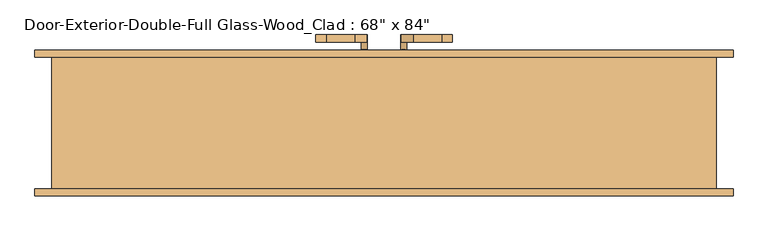
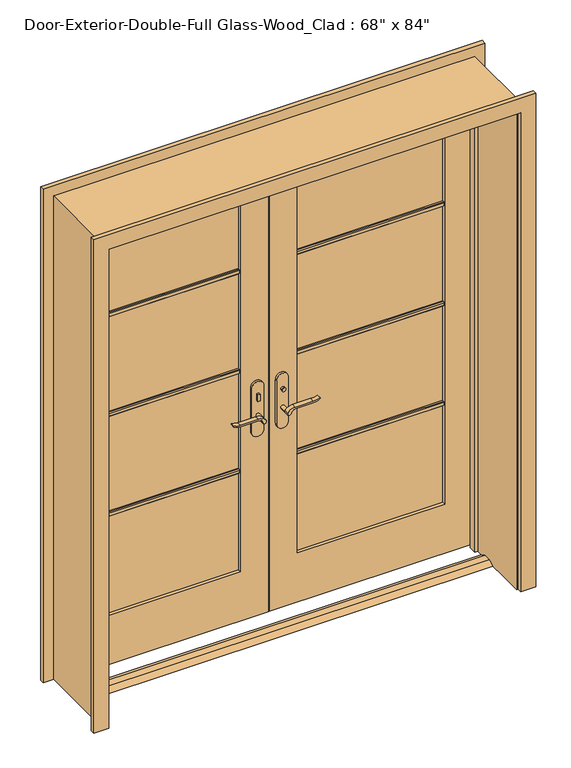
"""IFC4 building model written with IfcOpenShell, lengths in millimetres: door geometry."""

from ifc_helpers import new_model, si_unit, point, frame, frame_2d, origin, place, context, project, spatial, polyline, circle_curve, trimmed, segment, composite_curve, outline, extrude, faceted_brep, source, transform, mapped, element, save


def door_f2de18c9(model_context):
    return source(origin(), model_context, "Body", "SolidModel", [
        extrude(outline(polyline([(19.05, 12.7), (53.975, 12.7), (79.375, 0.0), (-6.35, 0.0), (19.05, 12.7)])), frame((-863.6, 0.0, 0.0), z_axis=(1.0, 0.0, 0.0), x_axis=(0.0, 1.0, 0.0)), (0.0, 0.0, 1.0), 1727.2),
        extrude(outline(polyline([(-47.4019111, 118.1125), (-57.4019111, 118.1125), (-57.4019111, 128.1125), (-47.4019111, 128.1125), (-47.4019111, 118.1125)])), frame((0.0, 0.0, 981.9), z_axis=(0.0, 0.0, 1.0), x_axis=(1.0, 0.0, 0.0)), (0.0, 0.0, 1.0), 30.0),
        extrude(outline(composite_curve([segment(trimmed(circle_curve(frame_2d((996.9, -52.4019111)), 8.0), [point((996.9, -60.4019111))], [point((996.9, -44.4019111))], False, "CARTESIAN"), True, "CONTINUOUS"), segment(trimmed(circle_curve(frame_2d((996.9, -52.4019111)), 8.0), [point((996.9, -44.4019111))], [point((996.9, -60.4019111))], False, "CARTESIAN"), True, "CONTINUOUS")], self_intersect=False)), frame((0.0, 183.0375, 0.0), z_axis=(0.0, 1.0, 0.0), x_axis=(0.0, 0.0, 1.0)), (0.0, 0.0, 1.0), 10.0),
        extrude(outline(composite_curve([segment(trimmed(circle_curve(frame_2d((897.1555521, -76.0694241)), 37.2832219), [point((919.0523287, -45.8937749))], [point((934.4, -77.7693445))], False, "CARTESIAN"), True, "CONTINUOUS"), segment(polyline([(934.4, -77.7693445), (934.4, -154.045502)]), True, "CONTINUOUS"), segment(trimmed(circle_curve(frame_2d((1017.6850638, -153.9791202)), 83.2850902), [point((934.4, -154.045502))], [point((939.4, -182.4019111))], True, "CARTESIAN"), True, "CONTINUOUS"), segment(polyline([(939.4, -182.4019111), (936.6135558, -182.4019111)]), True, "CONTINUOUS"), segment(trimmed(circle_curve(frame_2d((986.6709207, -150.4622499)), 59.3791355), [point((936.6135558, -182.4019111))], [point((927.4, -154.045502))], False, "CARTESIAN"), True, "CONTINUOUS"), segment(polyline([(927.4, -154.045502), (927.4, -77.7881013)]), True, "CONTINUOUS"), segment(trimmed(circle_curve(frame_2d((909.2738613, -77.7881013)), 18.1261387), [point((927.4, -77.7881013))], [point((914.4, -60.4019111))], True, "CARTESIAN"), True, "CONTINUOUS"), segment(trimmed(circle_curve(frame_2d((914.4, -52.4019111)), 8.0), [point((914.4, -60.4019111))], [point((919.0523287, -45.8937749))], False, "CARTESIAN"), True, "CONTINUOUS")], self_intersect=False)), frame((0.0, 78.1125, 0.0), z_axis=(0.0, 1.0, 0.0), x_axis=(0.0, 0.0, 1.0)), (0.0, 0.0, 1.0), 20.0),
        extrude(outline(composite_curve([segment(trimmed(circle_curve(frame_2d((914.4, -52.4019111)), 8.0), [point((914.3999903, -60.4019111))], [point((919.0523287, -45.8937749))], False, "CARTESIAN"), True, "CONTINUOUS"), segment(trimmed(circle_curve(frame_2d((897.1555521, -76.0694241)), 37.2832219), [point((919.0523287, -45.8937749))], [point((934.4, -77.7693445))], False, "CARTESIAN"), True, "CONTINUOUS"), segment(polyline([(934.4, -77.7693445), (934.4, -154.045502)]), True, "CONTINUOUS"), segment(trimmed(circle_curve(frame_2d((1017.6850638, -153.9791202)), 83.2850902), [point((934.4, -154.045502))], [point((939.4, -182.4019111))], True, "CARTESIAN"), True, "CONTINUOUS"), segment(polyline([(939.4, -182.4019111), (936.6135558, -182.4019111)]), True, "CONTINUOUS"), segment(trimmed(circle_curve(frame_2d((986.6709207, -150.4622499)), 59.3791355), [point((936.6135558, -182.4019111))], [point((927.4, -154.045502))], False, "CARTESIAN"), True, "CONTINUOUS"), segment(polyline([(927.4, -154.045502), (927.4, -77.788099)]), True, "CONTINUOUS"), segment(trimmed(circle_curve(frame_2d((909.2738682, -77.788099)), 18.1261318), [point((927.4, -77.788099))], [point((914.3999903, -60.4019111))], True, "CARTESIAN"), True, "CONTINUOUS")], self_intersect=False)), frame((0.0, 213.0375, 0.0), z_axis=(0.0, 1.0, 0.0), x_axis=(0.0, 0.0, 1.0)), (0.0, 0.0, 1.0), 20.0),
        extrude(outline(composite_curve([segment(trimmed(circle_curve(frame_2d((914.4, -52.4019111)), 8.0), [point((914.4, -60.4019111))], [point((914.4, -44.4019111))], False, "CARTESIAN"), True, "CONTINUOUS"), segment(trimmed(circle_curve(frame_2d((914.4, -52.4019111)), 8.0), [point((914.4, -44.4019111))], [point((914.4, -60.4019111))], False, "CARTESIAN"), True, "CONTINUOUS")], self_intersect=False)), frame((0.0, 98.1125, 0.0), z_axis=(0.0, 1.0, 0.0), x_axis=(0.0, 0.0, 1.0)), (0.0, 0.0, 1.0), 30.0),
        extrude(outline(composite_curve([segment(trimmed(circle_curve(frame_2d((914.4, -52.4019111)), 8.0), [point((914.4, -60.4019111))], [point((914.4, -44.4019111))], False, "CARTESIAN"), True, "CONTINUOUS"), segment(trimmed(circle_curve(frame_2d((914.4, -52.4019111)), 8.0), [point((914.4, -44.4019111))], [point((914.4, -60.4019111))], False, "CARTESIAN"), True, "CONTINUOUS")], self_intersect=False)), frame((0.0, 183.0375, 0.0), z_axis=(0.0, 1.0, 0.0), x_axis=(0.0, 0.0, 1.0)), (0.0, 0.0, 1.0), 30.0),
        extrude(outline(composite_curve([segment(polyline([(844.4, -27.4019111), (1039.4, -27.4019111)]), True, "CONTINUOUS"), segment(trimmed(circle_curve(frame_2d((1039.4, -52.4019111)), 25.0), [point((1039.4, -27.4019111))], [point((1039.4, -77.4019111))], False, "CARTESIAN"), True, "CONTINUOUS"), segment(polyline([(1039.4, -77.4019111), (844.4, -77.4019111)]), True, "CONTINUOUS"), segment(trimmed(circle_curve(frame_2d((844.4, -52.4019111)), 25.0), [point((844.4, -77.4019111))], [point((844.4, -27.4019111))], False, "CARTESIAN"), True, "CONTINUOUS")], self_intersect=False)), frame((0.0, 128.1125, 0.0), z_axis=(0.0, 1.0, 0.0), x_axis=(0.0, 0.0, 1.0)), (0.0, 0.0, 1.0), 10.0),
        extrude(outline(composite_curve([segment(polyline([(844.4, -27.4019111), (1039.4, -27.4019111)]), True, "CONTINUOUS"), segment(trimmed(circle_curve(frame_2d((1039.4, -52.4019111)), 25.0), [point((1039.4, -27.4019111))], [point((1039.4, -77.4019111))], False, "CARTESIAN"), True, "CONTINUOUS"), segment(polyline([(1039.4, -77.4019111), (844.4, -77.4019111)]), True, "CONTINUOUS"), segment(trimmed(circle_curve(frame_2d((844.4, -52.4019111)), 25.0), [point((844.4, -77.4019111))], [point((844.4, -27.4019111))], False, "CARTESIAN"), True, "CONTINUOUS")], self_intersect=False)), frame((0.0, 173.0375, 0.0), z_axis=(0.0, 1.0, 0.0), x_axis=(0.0, 0.0, 1.0)), (0.0, 0.0, 1.0), 10.0),
        extrude(outline(polyline([(47.3875, 193.0375), (57.3875, 193.0375), (57.3875, 183.0375), (47.3875, 183.0375), (47.3875, 193.0375)])), frame((0.0, 0.0, 981.9), z_axis=(0.0, 0.0, 1.0), x_axis=(1.0, 0.0, 0.0)), (0.0, 0.0, 1.0), 30.0),
        extrude(outline(composite_curve([segment(trimmed(circle_curve(frame_2d((996.9, 52.3875)), 8.0), [point((996.9, 60.3875))], [point((996.9, 44.3875))], False, "CARTESIAN"), True, "CONTINUOUS"), segment(trimmed(circle_curve(frame_2d((996.9, 52.3875)), 8.0), [point((996.9, 44.3875))], [point((996.9, 60.3875))], False, "CARTESIAN"), True, "CONTINUOUS")], self_intersect=False)), frame((0.0, 118.1125, 0.0), z_axis=(0.0, 1.0, 0.0), x_axis=(0.0, 0.0, 1.0)), (0.0, 0.0, 1.0), 10.0),
        extrude(outline(composite_curve([segment(trimmed(circle_curve(frame_2d((914.4, 52.3875)), 8.0), [point((919.0523287, 45.8793637))], [point((914.4, 60.3875))], False, "CARTESIAN"), True, "CONTINUOUS"), segment(trimmed(circle_curve(frame_2d((909.2738613, 77.7736901)), 18.1261387), [point((914.4, 60.3875))], [point((927.4, 77.7736901))], True, "CARTESIAN"), True, "CONTINUOUS"), segment(polyline([(927.4, 77.7736901), (927.4, 154.0310909)]), True, "CONTINUOUS"), segment(trimmed(circle_curve(frame_2d((986.6709207, 150.4478388)), 59.3791355), [point((927.4, 154.0310909))], [point((936.6135558, 182.3875))], False, "CARTESIAN"), True, "CONTINUOUS"), segment(polyline([(936.6135558, 182.3875), (939.4, 182.3875)]), True, "CONTINUOUS"), segment(trimmed(circle_curve(frame_2d((1017.6850638, 153.9647091)), 83.2850902), [point((939.4, 182.3875))], [point((934.4, 154.0310909))], True, "CARTESIAN"), True, "CONTINUOUS"), segment(polyline([(934.4, 154.0310909), (934.4, 77.7549333)]), True, "CONTINUOUS"), segment(trimmed(circle_curve(frame_2d((897.1555521, 76.0550129)), 37.2832219), [point((934.4, 77.7549333))], [point((919.0523287, 45.8793637))], False, "CARTESIAN"), True, "CONTINUOUS")], self_intersect=False)), frame((0.0, 213.0375, 0.0), z_axis=(0.0, 1.0, 0.0), x_axis=(0.0, 0.0, 1.0)), (0.0, 0.0, 1.0), 20.0),
        extrude(outline(composite_curve([segment(trimmed(circle_curve(frame_2d((909.2738682, 77.7736878)), 18.1261318), [point((914.3999903, 60.3875))], [point((927.4, 77.7736878))], True, "CARTESIAN"), True, "CONTINUOUS"), segment(polyline([(927.4, 77.7736878), (927.4, 154.0310909)]), True, "CONTINUOUS"), segment(trimmed(circle_curve(frame_2d((986.6709207, 150.4478388)), 59.3791355), [point((927.4, 154.0310909))], [point((936.6135558, 182.3875))], False, "CARTESIAN"), True, "CONTINUOUS"), segment(polyline([(936.6135558, 182.3875), (939.4, 182.3875)]), True, "CONTINUOUS"), segment(trimmed(circle_curve(frame_2d((1017.6850638, 153.9647091)), 83.2850902), [point((939.4, 182.3875))], [point((934.4, 154.0310909))], True, "CARTESIAN"), True, "CONTINUOUS"), segment(polyline([(934.4, 154.0310909), (934.4, 77.7549333)]), True, "CONTINUOUS"), segment(trimmed(circle_curve(frame_2d((897.1555521, 76.0550129)), 37.2832219), [point((934.4, 77.7549333))], [point((919.0523287, 45.8793637))], False, "CARTESIAN"), True, "CONTINUOUS"), segment(trimmed(circle_curve(frame_2d((914.4, 52.3875)), 8.0), [point((919.0523287, 45.8793637))], [point((914.3999903, 60.3875))], False, "CARTESIAN"), True, "CONTINUOUS")], self_intersect=False)), frame((0.0, 78.1125, 0.0), z_axis=(0.0, 1.0, 0.0), x_axis=(0.0, 0.0, 1.0)), (0.0, 0.0, 1.0), 20.0),
        extrude(outline(composite_curve([segment(trimmed(circle_curve(frame_2d((914.4, 52.3875)), 8.0), [point((914.4, 60.3875))], [point((914.4, 44.3875))], False, "CARTESIAN"), True, "CONTINUOUS"), segment(trimmed(circle_curve(frame_2d((914.4, 52.3875)), 8.0), [point((914.4, 44.3875))], [point((914.4, 60.3875))], False, "CARTESIAN"), True, "CONTINUOUS")], self_intersect=False)), frame((0.0, 183.0375, 0.0), z_axis=(0.0, 1.0, 0.0), x_axis=(0.0, 0.0, 1.0)), (0.0, 0.0, 1.0), 30.0),
        extrude(outline(composite_curve([segment(trimmed(circle_curve(frame_2d((914.4, 52.3875)), 8.0), [point((914.4, 60.3875))], [point((914.4, 44.3875))], False, "CARTESIAN"), True, "CONTINUOUS"), segment(trimmed(circle_curve(frame_2d((914.4, 52.3875)), 8.0), [point((914.4, 44.3875))], [point((914.4, 60.3875))], False, "CARTESIAN"), True, "CONTINUOUS")], self_intersect=False)), frame((0.0, 98.1125, 0.0), z_axis=(0.0, 1.0, 0.0), x_axis=(0.0, 0.0, 1.0)), (0.0, 0.0, 1.0), 30.0),
        extrude(outline(composite_curve([segment(trimmed(circle_curve(frame_2d((844.4, 52.3875)), 25.0), [point((844.4, 27.3875))], [point((844.4, 77.3875))], False, "CARTESIAN"), True, "CONTINUOUS"), segment(polyline([(844.4, 77.3875), (1039.4, 77.3875)]), True, "CONTINUOUS"), segment(trimmed(circle_curve(frame_2d((1039.4, 52.3875)), 25.0), [point((1039.4, 77.3875))], [point((1039.4, 27.3875))], False, "CARTESIAN"), True, "CONTINUOUS"), segment(polyline([(1039.4, 27.3875), (844.4, 27.3875)]), True, "CONTINUOUS")], self_intersect=False)), frame((0.0, 173.0375, 0.0), z_axis=(0.0, 1.0, 0.0), x_axis=(0.0, 0.0, 1.0)), (0.0, 0.0, 1.0), 10.0),
        extrude(outline(composite_curve([segment(trimmed(circle_curve(frame_2d((844.4, 52.3875)), 25.0), [point((844.4, 27.3875))], [point((844.4, 77.3875))], False, "CARTESIAN"), True, "CONTINUOUS"), segment(polyline([(844.4, 77.3875), (1039.4, 77.3875)]), True, "CONTINUOUS"), segment(trimmed(circle_curve(frame_2d((1039.4, 52.3875)), 25.0), [point((1039.4, 77.3875))], [point((1039.4, 27.3875))], False, "CARTESIAN"), True, "CONTINUOUS"), segment(polyline([(1039.4, 27.3875), (844.4, 27.3875)]), True, "CONTINUOUS")], self_intersect=False)), frame((0.0, 128.1125, 0.0), z_axis=(0.0, 1.0, 0.0), x_axis=(0.0, 0.0, 1.0)), (0.0, 0.0, 1.0), 10.0),
        extrude(outline(polyline([(152.0825, 1578.371875), (152.0825, 1559.321875), (145.7325, 1559.321875), (142.5575, 1562.496875), (142.5575, 1575.196875), (145.7325, 1578.371875), (152.0825, 1578.371875)])), frame((120.65, 0.0, 0.0), z_axis=(1.0, 0.0, 0.0), x_axis=(0.0, 1.0, 0.0)), (0.0, 0.0, 1.0), 622.3),
        extrude(outline(polyline([(152.0825, 1132.68125), (152.0825, 1113.63125), (145.7325, 1113.63125), (142.5575, 1116.80625), (142.5575, 1129.50625), (145.7325, 1132.68125), (152.0825, 1132.68125)])), frame((120.65, 0.0, 0.0), z_axis=(1.0, 0.0, 0.0), x_axis=(0.0, 1.0, 0.0)), (0.0, 0.0, 1.0), 622.3),
        extrude(outline(polyline([(152.0825, 686.990625), (152.0825, 667.940625), (145.7325, 667.940625), (142.5575, 671.115625), (142.5575, 683.815625), (145.7325, 686.990625), (152.0825, 686.990625)])), frame((120.65, 0.0, 0.0), z_axis=(1.0, 0.0, 0.0), x_axis=(0.0, 1.0, 0.0)), (0.0, 0.0, 1.0), 622.3),
        extrude(outline(polyline([(159.0675, 1578.371875), (165.4175, 1578.371875), (168.5925, 1575.196875), (168.5925, 1562.496875), (165.4175, 1559.321875), (159.0675, 1559.321875), (159.0675, 1578.371875)])), frame((-742.95, 0.0, 0.0), z_axis=(1.0, 0.0, 0.0), x_axis=(0.0, 1.0, 0.0)), (0.0, 0.0, 1.0), 622.3),
        extrude(outline(polyline([(159.0675, 1132.68125), (165.4175, 1132.68125), (168.5925, 1129.50625), (168.5925, 1116.80625), (165.4175, 1113.63125), (159.0675, 1113.63125), (159.0675, 1132.68125)])), frame((-742.95, 0.0, 0.0), z_axis=(1.0, 0.0, 0.0), x_axis=(0.0, 1.0, 0.0)), (0.0, 0.0, 1.0), 622.3),
        extrude(outline(polyline([(159.0675, 686.990625), (165.4175, 686.990625), (168.5925, 683.815625), (168.5925, 671.115625), (165.4175, 667.940625), (159.0675, 667.940625), (159.0675, 686.990625)])), frame((-742.95, 0.0, 0.0), z_axis=(1.0, 0.0, 0.0), x_axis=(0.0, 1.0, 0.0)), (0.0, 0.0, 1.0), 622.3),
        extrude(outline(polyline([(159.0675, 1578.371875), (165.4175, 1578.371875), (168.5925, 1575.196875), (168.5925, 1562.496875), (165.4175, 1559.321875), (159.0675, 1559.321875), (159.0675, 1578.371875)])), frame((120.65, 0.0, 0.0), z_axis=(1.0, 0.0, 0.0), x_axis=(0.0, 1.0, 0.0)), (0.0, 0.0, 1.0), 622.3),
        extrude(outline(polyline([(159.0675, 1132.68125), (165.4175, 1132.68125), (168.5925, 1129.50625), (168.5925, 1116.80625), (165.4175, 1113.63125), (159.0675, 1113.63125), (159.0675, 1132.68125)])), frame((120.65, 0.0, 0.0), z_axis=(1.0, 0.0, 0.0), x_axis=(0.0, 1.0, 0.0)), (0.0, 0.0, 1.0), 622.3),
        extrude(outline(polyline([(159.0675, 686.990625), (165.4175, 686.990625), (168.5925, 683.815625), (168.5925, 671.115625), (165.4175, 667.940625), (159.0675, 667.940625), (159.0675, 686.990625)])), frame((120.65, 0.0, 0.0), z_axis=(1.0, 0.0, 0.0), x_axis=(0.0, 1.0, 0.0)), (0.0, 0.0, 1.0), 622.3),
        extrude(outline(polyline([(152.0825, 1578.371875), (152.0825, 1559.321875), (145.7325, 1559.321875), (142.5575, 1562.496875), (142.5575, 1575.196875), (145.7325, 1578.371875), (152.0825, 1578.371875)])), frame((-742.95, 0.0, 0.0), z_axis=(1.0, 0.0, 0.0), x_axis=(0.0, 1.0, 0.0)), (0.0, 0.0, 1.0), 622.3),
        extrude(outline(polyline([(152.0825, 1132.68125), (152.0825, 1113.63125), (145.7325, 1113.63125), (142.5575, 1116.80625), (142.5575, 1129.50625), (145.7325, 1132.68125), (152.0825, 1132.68125)])), frame((-742.95, 0.0, 0.0), z_axis=(1.0, 0.0, 0.0), x_axis=(0.0, 1.0, 0.0)), (0.0, 0.0, 1.0), 622.3),
        extrude(outline(polyline([(152.0825, 686.990625), (152.0825, 667.940625), (145.7325, 667.940625), (142.5575, 671.115625), (142.5575, 683.815625), (145.7325, 686.990625), (152.0825, 686.990625)])), frame((-742.95, 0.0, 0.0), z_axis=(1.0, 0.0, 0.0), x_axis=(0.0, 1.0, 0.0)), (0.0, 0.0, 1.0), 622.3),
        extrude(outline(polyline([(0.0, 869.95), (0.0, 933.45), (2203.45, 933.45), (2203.45, -933.45), (0.0, -933.45), (0.0, -869.95), (2139.95, -869.95), (2139.95, 869.95), (0.0, 869.95)])), frame((0.0, 173.0375, 0.0), z_axis=(0.0, 1.0, 0.0), x_axis=(0.0, 0.0, 1.0)), (0.0, 0.0, 1.0), 19.05),
        extrude(outline(polyline([(0.0, 869.95), (0.0, 933.45), (2203.45, 933.45), (2203.45, -933.45), (0.0, -933.45), (0.0, -869.95), (2139.95, -869.95), (2139.95, 869.95), (0.0, 869.95)])), frame((0.0, -198.4375, 0.0), z_axis=(0.0, 1.0, 0.0), x_axis=(0.0, 0.0, 1.0)), (0.0, 0.0, 1.0), 19.05),
        extrude(outline(polyline([(12.7, 863.6), (2133.6, 863.6), (2133.6, 1.5875), (12.7, 1.5875), (12.7, 863.6)]), holes=[polyline([(2014.5375, 120.65), (2014.5375, 742.95), (231.775, 742.95), (231.775, 120.65), (2014.5375, 120.65)])]), frame((0.0, 138.1125, 0.0), z_axis=(0.0, 1.0, 0.0), x_axis=(0.0, 0.0, 1.0)), (0.0, 0.0, 1.0), 34.925),
        extrude(outline(polyline([(2133.6, -863.6), (12.7, -863.6), (12.7, -1.6019111), (2133.6, -1.6019111), (2133.6, -863.6)]), holes=[polyline([(231.775, -742.95), (2014.5375, -742.95), (2014.5375, -120.65), (231.775, -120.65), (231.775, -742.95)])]), frame((0.0, 138.1125, 0.0), z_axis=(0.0, 1.0, 0.0), x_axis=(0.0, 0.0, 1.0)), (0.0, 0.0, 1.0), 34.925),
        faceted_brep([(889.0, 173.0375, 0.0), (889.0, -179.3875, 0.0), (863.6, -179.3875, 0.0), (863.6, 103.1875, 0.0), (850.9, 103.1875, 0.0), (850.9, 138.1125, 0.0), (863.6, 138.1125, 0.0), (863.6, 173.0375, 0.0), (889.0, 173.0375, 2159.0), (889.0, -179.3875, 2159.0), (-889.0, -179.3875, 2159.0), (-889.0, -179.3875, 0.0), (-863.6, -179.3875, 0.0), (-863.6, -179.3875, 2133.6), (863.6, -179.3875, 2133.6), (863.6, 103.1875, 2133.6), (-863.6, 103.1875, 2133.6), (-863.6, 103.1875, 0.0), (-850.9, 103.1875, 0.0), (-850.9, 103.1875, 2120.9), (850.9, 103.1875, 2120.9), (850.9, 138.1125, 2120.9), (1.5875, 138.1125, 2120.9), (-1.6019111, 138.1125, 2120.9), (-850.9, 138.1125, 2120.9), (-850.9, 138.1125, 0.0), (-863.6, 138.1125, 0.0), (-863.6, 138.1125, 2133.6), (-1.6019111, 138.1125, 2133.6), (1.5875, 138.1125, 2133.6), (863.6, 138.1125, 2133.6), (863.6, 173.0375, 2133.6), (1.5875, 173.0375, 2133.6), (-1.6019111, 173.0375, 2133.6), (-863.6, 173.0375, 2133.6), (-863.6, 173.0375, 0.0), (-889.0, 173.0375, 0.0), (-889.0, 173.0375, 2159.0)], [[[0, 1, 2, 3, 4, 5, 6, 7]], [[1, 0, 8, 9]], [[2, 1, 9, 10, 11, 12, 13, 14]], [[3, 2, 14, 15]], [[4, 3, 15, 16, 17, 18, 19, 20]], [[5, 4, 20, 21]], [[6, 5, 21, 22, 23, 24, 25, 26, 27, 28, 29, 30]], [[7, 6, 30, 31]], [[0, 7, 31, 32, 33, 34, 35, 36, 37, 8]], [[9, 8, 37, 10]], [[14, 13, 16, 15]], [[20, 19, 24, 23, 22, 21]], [[31, 30, 29, 28, 27, 34, 33, 32]], [[12, 11, 36, 35, 26, 25, 18, 17]], [[11, 10, 37, 36]], [[13, 12, 17, 16]], [[19, 18, 25, 24]], [[27, 26, 35, 34]]]),
        extrude(outline(polyline([(742.95, 152.0825), (120.65, 152.0825), (120.65, 159.0675), (742.95, 159.0675), (742.95, 152.0825)])), frame((0.0, 0.0, 231.775), z_axis=(0.0, 0.0, 1.0), x_axis=(1.0, 0.0, 0.0)), (0.0, 0.0, 1.0), 1782.7625),
        extrude(outline(polyline([(-120.65, 152.0825), (-742.95, 152.0825), (-742.95, 159.0675), (-120.65, 159.0675), (-120.65, 152.0825)])), frame((0.0, 0.0, 231.775), z_axis=(0.0, 0.0, 1.0), x_axis=(1.0, 0.0, 0.0)), (0.0, 0.0, 1.0), 1782.7625),
    ])


if __name__ == "__main__":
    model = new_model("IFC4")
    model_context = context("Model", 3, world=origin())
    ifc_project = project(units=[si_unit("LENGTHUNIT", "METRE", prefix="MILLI")], contexts=[model_context])
    site = spatial("IfcSite", under=ifc_project)
    building = spatial("IfcBuilding", under=site)
    placement = place(None, origin())
    door_shape = door_f2de18c9(model_context)
    element("IfcDoor", 1, ObjectType="Door-Exterior-Double-Full Glass-Wood_Clad : 68\" x 84\"", at=placement, inside=building, context=model_context, shape_type="MappedRepresentation", body=[
        mapped(door_shape, transform((0.0, 0.0, 0.0), x_axis=(1.0, 0.0, 0.0), y_axis=(0.0, 1.0, 0.0), z_axis=(0.0, 0.0, 1.0))),
    ])
    save(model, "model.ifc")

# Revit data of these elements
# Type "Door-Exterior-Double-Full Glass-Wood_Clad : 68\" x 84\""
#   Type Mark = "12"
#   Assembly Code = "B2030100"
#   Analytic Construction = "French door, wood frame with double glass"
#   Top Rail = 0' - 4 11/16"
#   Threshold Offset [instance default] = 0' - 0 1/2"
#   Thickness = 0' - 1 3/8"
#   Thermal Resistance (R) = 1.9158 (h·ft²·°F)/BTU
#   Swing Angle [instance default] = 90.00°
#   Stiles = 0' - 4 3/4"
#   Rough Width = 5' - 10"
#   Rough Height = 7' - 1"
#   Panel Width = 2' - 10"
#   Door Offset [instance default] = 0' - 0"
#   Height = 7' - 0"
#   Width = 5' - 8"
#   Heat Transfer Coefficient (U) = 0.5220 BTU/(h·ft²·°F)
#   Bottom Rail = 0' - 9 1/8"
#   Exterior Trim [instance default] = yes
#   Threshold [instance default] = yes
#   Show Grill [instance default] = yes
#   Function = 1
#   Trim Material = Cherry
#   Threshold Material = Cherry
#   Panel Material = Cherry
#   Glazing = Glass
#   Frame Material = Cherry
#   Door Handle Material = Aluminum
#   Visual Light Transmittance = 0
#   Solar Heat Gain Coefficient = 0
#   Wall Closure = (empty or 0)
#   Construction Type = (empty or 0)
# Element 1 (IfcDoor, "Door-Exterior-Double-Full Glass-Wood_Clad : 68\" x 84\"")
#   Materials on its faces: "Cherry", "Aluminum", "Glass"
# Materials
#   "Cherry": class "Wood", colour RGB 226 177 128, transparency 0, Description = "Prunus Serotina", Cost = 0
#   "Glass": class "Glass", colour RGB 0 128 192, transparency 0.75, Description = "Soda Lime Glass", Cost = 0
#   "Aluminum": class "Metal", colour RGB 247 247 247, transparency 0, Description = "Aluminum 6061", Cost = 0
